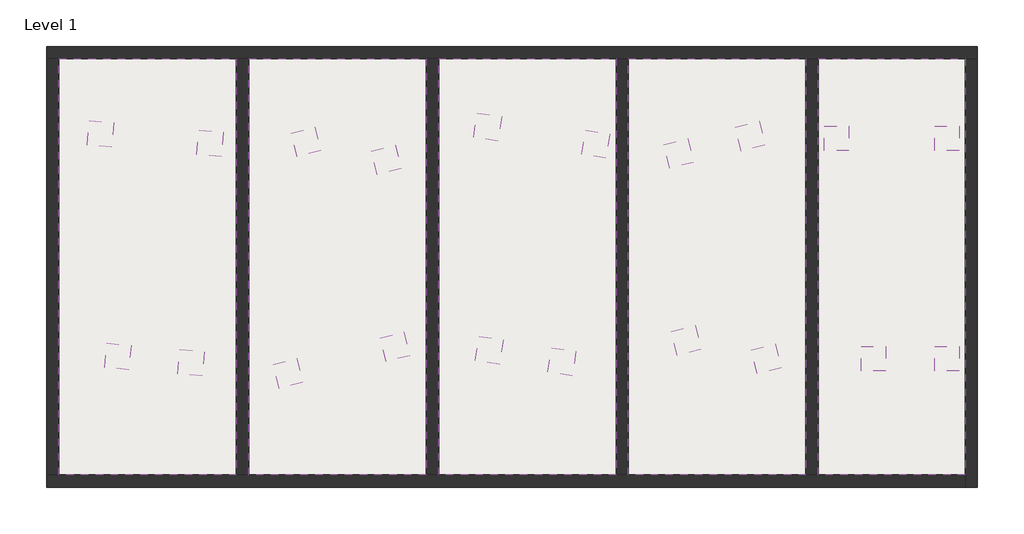
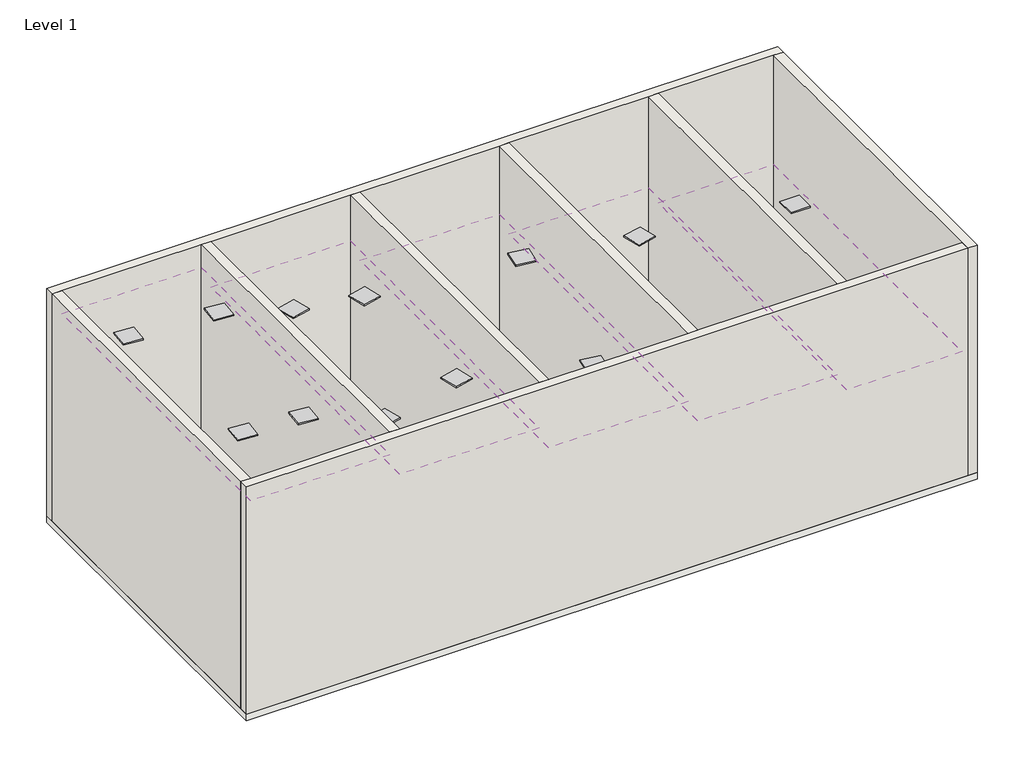
# One storey: 20 light fixtures, 8 walls, 5 coverings, 1 slab.
"""IFC4 building model written with IfcOpenShell, lengths in millimetres."""

import ifcopenshell
import ifcopenshell.guid

model = None  # the IFC model being written
_history = None  # IfcOwnerHistory: only IFC2X3 demands one
_inside = {}  # id of a spatial element -> (the spatial element, [elements in it])
_under = {}  # id of a project, library or spatial element -> (it, [spatial elements below it])
_declared = {}  # id of a project -> (the project, [libraries it declares])
_typed = {}  # id of a type object -> (the type object, [elements of that type])
_made_of = {}  # id of a material, layer set ... -> (it, [elements and type objects made of it])


def new_model(schema):
    """Start an empty IFC model of exactly this schema.

    Asked for "IFC4X3", IfcOpenShell would pick the latest addendum, in which some entities
    have other attributes; the version numbers below select the first issue.
    IFC2X3 requires an IfcOwnerHistory on every rooted entity: one is made here for all.
    """
    global model, _history
    if schema == "IFC4X3":
        model = ifcopenshell.file(schema_version=(4, 3, 0, 0))
    else:
        model = ifcopenshell.file(schema=schema)
    _inside.clear()
    _under.clear()
    _declared.clear()
    _typed.clear()
    _made_of.clear()
    _history = None
    if model.schema == "IFC2X3":
        org = make("IfcOrganization", Name="unknown")
        user = make(
            "IfcPersonAndOrganization",
            ThePerson=make("IfcPerson", FamilyName="unknown"),
            TheOrganization=org,
        )
        app = make(
            "IfcApplication",
            ApplicationDeveloper=org,
            Version="unknown",
            ApplicationFullName="unknown",
            ApplicationIdentifier="unknown",
        )
        _history = make(
            "IfcOwnerHistory",
            OwningUser=user,
            OwningApplication=app,
            ChangeAction="ADDED",
            CreationDate=0,
        )
    return model


def make(cls, **values):
    """One entity of the class cls with the attributes given. An attribute that is None is left unset."""
    return model.create_entity(
        cls, **{name: value for name, value in values.items() if value is not None}
    )


def rooted(cls, **values):
    """An entity with a GlobalId (a new one), such as an element, a storey or a relation."""
    return make(cls, GlobalId=ifcopenshell.guid.new(), OwnerHistory=_history, **values)


def si_unit(unit_type, name, prefix=None):
    """IfcSIUnit, for example si_unit("LENGTHUNIT", "METRE", prefix="MILLI")."""
    return make("IfcSIUnit", UnitType=unit_type, Prefix=prefix, Name=name)


def assignment(units):
    """IfcUnitAssignment: the units of a project."""
    return None if units is None else make("IfcUnitAssignment", Units=units)


def point(xyz):
    """IfcCartesianPoint."""
    return None if xyz is None else make("IfcCartesianPoint", Coordinates=xyz)


def direction(xyz):
    """IfcDirection."""
    return None if xyz is None else make("IfcDirection", DirectionRatios=xyz)


def frame(location, z_axis=None, x_axis=None):
    """IfcAxis2Placement3D, a coordinate frame: its origin and axes. An axis left out is left unset."""
    return make(
        "IfcAxis2Placement3D",
        Location=point(location),
        Axis=direction(z_axis),
        RefDirection=direction(x_axis),
    )


def origin():
    """The frame at (0, 0, 0) with its axes left unset."""
    return frame((0.0, 0.0, 0.0))


def origin_with_axes():
    """The frame at (0, 0, 0) with the z axis (0, 0, 1) and the x axis (1, 0, 0) written out."""
    return frame((0.0, 0.0, 0.0), z_axis=(0.0, 0.0, 1.0), x_axis=(1.0, 0.0, 0.0))


def place(relative_to, where):
    """IfcLocalPlacement: puts the frame where relative to a parent placement (None: the world)."""
    return make(
        "IfcLocalPlacement", PlacementRelTo=relative_to, RelativePlacement=where
    )


def context(
    kind, dimensions, precision=None, world=None, true_north=None, identifier=None
):
    """IfcGeometricRepresentationContext, for example the 3D "Model" context."""
    return make(
        "IfcGeometricRepresentationContext",
        ContextIdentifier=identifier,
        ContextType=kind,
        CoordinateSpaceDimension=dimensions,
        Precision=precision,
        WorldCoordinateSystem=world,
        TrueNorth=true_north,
    )


def project(units=None, contexts=None):
    """IfcProject with its units and contexts."""
    return rooted(
        "IfcProject",
        Name="project",
        RepresentationContexts=contexts,
        UnitsInContext=assignment(units),
    )


def spatial(cls, under=None, at=None, **own):
    """A site, building, storey or space (cls), placed at a placement, below another one or the project."""
    s = rooted(cls, ObjectPlacement=at, **own)
    if under is not None:
        _under.setdefault(under.id(), (under, []))[1].append(s)
    return s


def polyline(points):
    """IfcPolyline through the points."""
    return make("IfcPolyline", Points=[point(p) for p in points])


def outline(outer, holes=None, kind="AREA"):
    """IfcArbitraryClosedProfileDef: a profile drawn as a closed curve; with holes, ...WithVoids."""
    if holes is None:
        return make("IfcArbitraryClosedProfileDef", ProfileType=kind, OuterCurve=outer)
    return make(
        "IfcArbitraryProfileDefWithVoids",
        ProfileType=kind,
        OuterCurve=outer,
        InnerCurves=holes,
    )


def extrude(swept, where, along, depth):
    """IfcExtrudedAreaSolid: the profile swept, set in the frame where, extruded along a direction by depth."""
    return make(
        "IfcExtrudedAreaSolid",
        SweptArea=swept,
        Position=where,
        ExtrudedDirection=direction(along),
        Depth=depth,
    )


def faces_of(points, faces, orient=None, outer=None):
    """IfcFace entities. A face is a list of loops; a loop is a list of indices into points, from 0.

    orient and outer hold one flag for each loop. By default every Orientation is true, the
    first loop of a face is its IfcFaceOuterBound and the others are IfcFaceBound.
    """
    made = []
    for i, loops in enumerate(faces):
        bounds = []
        for j, loop in enumerate(loops):
            is_outer = j == 0 if outer is None else outer[i][j]
            bounds.append(
                make(
                    "IfcFaceOuterBound" if is_outer else "IfcFaceBound",
                    Bound=make("IfcPolyLoop", Polygon=[points[k] for k in loop]),
                    Orientation=True if orient is None else orient[i][j],
                )
            )
        made.append(make("IfcFace", Bounds=bounds))
    return made


def faceted_brep(points, faces, orient=None, outer=None, voids=None):
    """IfcFacetedBrep: a solid bounded by flat faces; with voids (closed shells), ...WithVoids."""
    shared = [point(p) for p in points]
    hull = make("IfcClosedShell", CfsFaces=faces_of(shared, faces, orient, outer))
    if voids is None:
        return make("IfcFacetedBrep", Outer=hull)
    return make(
        "IfcFacetedBrepWithVoids",
        Outer=hull,
        Voids=[
            make(cls, CfsFaces=faces_of(shared, fs, o, b)) for cls, fs, o, b in voids
        ],
    )


def shape(context_of_items, identifier, shape_type, items):
    """IfcShapeRepresentation: the items that make up one representation, for example the "Body"."""
    return make(
        "IfcShapeRepresentation",
        ContextOfItems=context_of_items,
        RepresentationIdentifier=identifier,
        RepresentationType=shape_type,
        Items=items,
    )


def source(mapping_origin, context_of_items, identifier, shape_type, items):
    """IfcRepresentationMap: a shape defined once, which mapped items show again and again."""
    return make(
        "IfcRepresentationMap",
        MappingOrigin=mapping_origin,
        MappedRepresentation=shape(context_of_items, identifier, shape_type, items),
    )


def transform(
    local_origin,
    x_axis=None,
    y_axis=None,
    z_axis=None,
    scale=None,
    scale2=None,
    scale3=None,
    uniform=True,
):
    """IfcCartesianTransformationOperator3D, or its non-uniform kind. x_axis, y_axis, z_axis: its Axis1, 2, 3."""
    if uniform:
        return make(
            "IfcCartesianTransformationOperator3D",
            Axis1=direction(x_axis),
            Axis2=direction(y_axis),
            LocalOrigin=point(local_origin),
            Scale=scale,
            Axis3=direction(z_axis),
        )
    return make(
        "IfcCartesianTransformationOperator3DnonUniform",
        Axis1=direction(x_axis),
        Axis2=direction(y_axis),
        LocalOrigin=point(local_origin),
        Scale=scale,
        Axis3=direction(z_axis),
        Scale2=scale2,
        Scale3=scale3,
    )


def mapped(mapping_source, mapping_target):
    """IfcMappedItem: shows the shape of a source again, moved by a transform."""
    return make(
        "IfcMappedItem", MappingSource=mapping_source, MappingTarget=mapping_target
    )


def made_of(thing, what):
    """Note that an element or type object is made of a material, layer set ...; save() writes the relation."""
    if what is not None:
        _made_of.setdefault(what.id(), (what, []))[1].append(thing)
    return thing


def element(
    cls,
    number,
    at=None,
    inside=None,
    cuts=None,
    type_object=None,
    material=None,
    context=None,
    identifier="Body",
    shape_type=None,
    held_by="IfcProductDefinitionShape",
    body=None,
    shapes=None,
    **own,
):
    """One element of the class cls, such as IfcWall. Its Tag is "e" and its number.

    at: its placement. inside: the storey or other place that contains it. cuts: it is an
    opening in that element (IfcRelVoidsElement). A single representation is given by context,
    identifier, shape_type and body (its items); several are given by shapes. held_by: the class
    of the entity that holds the representations. save() writes the other relations.
    """
    e = rooted(cls, Tag="e%d" % number, ObjectPlacement=at, **own)
    if body is not None:
        shapes = [shape(context, identifier, shape_type, body)]
    if shapes is not None:
        e.Representation = make(held_by, Representations=shapes)
    if inside is not None:
        _inside.setdefault(inside.id(), (inside, []))[1].append(e)
    if cuts is not None:
        rooted(
            "IfcRelVoidsElement", RelatingBuildingElement=cuts, RelatedOpeningElement=e
        )
    if type_object is not None:
        _typed.setdefault(type_object.id(), (type_object, []))[1].append(e)
    return made_of(e, material)


def aggregate(whole, parts):
    """IfcRelAggregates: a whole, such as a stair, and the parts it consists of."""
    return rooted("IfcRelAggregates", RelatingObject=whole, RelatedObjects=parts)


def save(model, path):
    """Write the relations noted so far, then the file.

    IfcRelAggregates (storeys below a building ...), IfcRelContainedInSpatialStructure (elements
    in a storey), IfcRelDefinesByType, IfcRelAssociatesMaterial and IfcRelDeclares: one each for
    every whole, place, type object, material and project.
    """
    for whole, parts in _under.values():
        aggregate(whole, parts)
    for where, things in _inside.values():
        rooted(
            "IfcRelContainedInSpatialStructure",
            RelatedElements=things,
            RelatingStructure=where,
        )
    for kind, things in _typed.values():
        rooted("IfcRelDefinesByType", RelatedObjects=things, RelatingType=kind)
    for what, things in _made_of.values():
        rooted("IfcRelAssociatesMaterial", RelatedObjects=things, RelatingMaterial=what)
    for by, libraries in _declared.values():
        rooted("IfcRelDeclares", RelatingContext=by, RelatedDefinitions=libraries)
    model.write(path)


def downlight_downlight_20077eaa(model_context):
    return source(origin(), model_context, "Body", "SweptSolid", [
        extrude(outline(polyline([(200.0, -200.0), (-200.0, -200.0), (-200.0, 200.0), (200.0, 200.0), (200.0, -200.0)])), frame((0.0, 0.0, -4.6872227), z_axis=(0.0, 0.0, 1.0), x_axis=(1.0, 0.0, 0.0)), (0.0, 0.0, 1.0), 24.9370919),
    ])


model = new_model("IFC4")

# Units and contexts
model_context = context("Model", 3, world=origin())
ifc_project = project(units=[si_unit("LENGTHUNIT", "METRE", prefix="MILLI")], contexts=[model_context])

# Site, building, storey
site = spatial("IfcSite", under=ifc_project)
building = spatial("IfcBuilding", under=site)
storey = spatial("IfcBuildingStorey", under=building, Name="Level 1", Elevation=0.0)

# Coverings
placement = place(None, origin())
element("IfcCovering", 1, ObjectType="600 x 600mm Grid", at=placement, inside=storey, context=model_context, shape_type="SweptSolid", body=[
    extrude(outline(polyline([(4711.6370984, -2494.7382368), (4711.6370984, 4305.2617632), (7111.6370984, 4305.2617632), (7111.6370984, -2494.7382368), (4711.6370984, -2494.7382368)])), frame((0.0, 0.0, 2600.0), z_axis=(0.0, 0.0, 1.0), x_axis=(1.0, 0.0, 0.0)), (0.0, 0.0, 1.0), 52.0),
])
element("IfcCovering", 2, ObjectType="600 x 600mm Grid", at=placement, inside=storey, context=model_context, shape_type="SweptSolid", body=[
    extrude(outline(polyline([(1611.6370984, -2494.7382368), (1611.6370984, 4305.2617632), (4511.6370984, 4305.2617632), (4511.6370984, -2494.7382368), (1611.6370984, -2494.7382368)])), frame((0.0, 0.0, 3000.0), z_axis=(0.0, 0.0, 1.0), x_axis=(1.0, 0.0, 0.0)), (0.0, 0.0, 1.0), 52.0),
])
element("IfcCovering", 3, ObjectType="600 x 600mm Grid", at=placement, inside=storey, context=model_context, shape_type="SweptSolid", body=[
    extrude(outline(polyline([(-1488.3629016, -2494.7382368), (-1488.3629016, 4305.2617632), (1411.6370984, 4305.2617632), (1411.6370984, -2494.7382368), (-1488.3629016, -2494.7382368)])), frame((0.0, 0.0, 3500.0), z_axis=(0.0, 0.0, 1.0), x_axis=(1.0, 0.0, 0.0)), (0.0, 0.0, 1.0), 52.0),
])
element("IfcCovering", 4, ObjectType="600 x 600mm Grid", at=placement, inside=storey, context=model_context, shape_type="SweptSolid", body=[
    extrude(outline(polyline([(-4588.3629016, -2494.7382368), (-4588.3629016, 4305.2617632), (-1688.3629016, 4305.2617632), (-1688.3629016, -2494.7382368), (-4588.3629016, -2494.7382368)])), frame((0.0, 0.0, 4000.0), z_axis=(0.0, 0.0, 1.0), x_axis=(1.0, 0.0, 0.0)), (0.0, 0.0, 1.0), 52.0),
])
element("IfcCovering", 5, ObjectType="600 x 600mm Grid", at=placement, inside=storey, context=model_context, shape_type="SweptSolid", body=[
    extrude(outline(polyline([(-7688.3629016, 4305.2617632), (-4788.3629016, 4305.2617632), (-4788.3629016, -2494.7382368), (-7688.3629016, -2494.7382368), (-7688.3629016, 4305.2617632)])), frame((0.0, 0.0, 4500.0), z_axis=(0.0, 0.0, 1.0), x_axis=(1.0, 0.0, 0.0)), (0.0, 0.0, 1.0), 52.0),
])

# Light fixtures
downlight_downlight_shape = downlight_downlight_20077eaa(model_context)
element("IfcLightFixture", 6, ObjectType="Downlight : Downlight", at=placement, inside=storey, context=model_context, shape_type="MappedRepresentation", body=[
    mapped(downlight_downlight_shape, transform((-7009.3072235, 3078.2167678, 4500.0), x_axis=(0.9961946980917439, -0.08715574274767758, 0.0), y_axis=(0.08715574274767758, 0.9961946980917439, 0.0), z_axis=(0.0, 0.0, 1.0))),
])
element("IfcLightFixture", 7, ObjectType="Downlight : Downlight", at=placement, inside=storey, context=model_context, shape_type="MappedRepresentation", body=[
    mapped(downlight_downlight_shape, transform((-5216.1567669, 2921.3364309, 4500.0), x_axis=(0.9961946980917439, -0.08715574274767879, 0.0), y_axis=(0.08715574274767879, 0.9961946980917439, 0.0), z_axis=(0.0, 0.0, 1.0))),
])
element("IfcLightFixture", 8, ObjectType="Downlight : Downlight", at=placement, inside=storey, context=model_context, shape_type="MappedRepresentation", body=[
    mapped(downlight_downlight_shape, transform((-5529.9174408, -664.9644822, 4500.0), x_axis=(0.9961946980917413, -0.08715574274770704, 0.0), y_axis=(0.08715574274770704, 0.9961946980917413, 0.0), z_axis=(0.0, 0.0, 1.0))),
])
element("IfcLightFixture", 9, ObjectType="Downlight : Downlight", at=placement, inside=storey, context=model_context, shape_type="MappedRepresentation", body=[
    mapped(downlight_downlight_shape, transform((-6725.3510785, -560.3775909, 4500.0), x_axis=(0.9961946980917413, -0.08715574274770621, 0.0), y_axis=(0.08715574274770621, 0.9961946980917413, 0.0), z_axis=(0.0, 0.0, 1.0))),
])
element("IfcLightFixture", 10, ObjectType="Downlight : Downlight", at=placement, inside=storey, context=model_context, shape_type="MappedRepresentation", body=[
    mapped(downlight_downlight_shape, transform((-3651.9813594, 2945.0444871, 4000.0), x_axis=(0.24192189559968028, -0.9702957262759934, 0.0), y_axis=(0.9702957262759934, 0.24192189559968028, 0.0), z_axis=(0.0, 0.0, 1.0))),
])
element("IfcLightFixture", 11, ObjectType="Downlight : Downlight", at=placement, inside=storey, context=model_context, shape_type="MappedRepresentation", body=[
    mapped(downlight_downlight_shape, transform((-2342.4733505, 2653.173326, 4000.0), x_axis=(0.24192189559967206, -0.9702957262759955, 0.0), y_axis=(0.9702957262759955, 0.24192189559967206, 0.0), z_axis=(0.0, 0.0, 1.0))),
])
element("IfcLightFixture", 12, ObjectType="Downlight : Downlight", at=placement, inside=storey, context=model_context, shape_type="MappedRepresentation", body=[
    mapped(downlight_downlight_shape, transform((-2198.8850995, -402.8669901, 4000.0), x_axis=(0.24192189559958152, -0.970295726276018, 0.0), y_axis=(0.970295726276018, 0.24192189559958152, 0.0), z_axis=(0.0, 0.0, 1.0))),
])
element("IfcLightFixture", 13, ObjectType="Downlight : Downlight", at=placement, inside=storey, context=model_context, shape_type="MappedRepresentation", body=[
    mapped(downlight_downlight_shape, transform((-3945.4174068, -838.3264022, 4000.0), x_axis=(0.241921895599675, -0.9702957262759947, 0.0), y_axis=(0.9702957262759947, 0.241921895599675, 0.0), z_axis=(0.0, 0.0, 1.0))),
])
element("IfcLightFixture", 14, ObjectType="Downlight : Downlight", at=placement, inside=storey, context=model_context, shape_type="MappedRepresentation", body=[
    mapped(downlight_downlight_shape, transform((-687.666432, 3190.6624322, 3500.0), x_axis=(0.9876883405951378, -0.15643446504023112, 0.0), y_axis=(0.15643446504023112, 0.9876883405951378, 0.0), z_axis=(0.0, 0.0, 1.0))),
])
element("IfcLightFixture", 15, ObjectType="Downlight : Downlight", at=placement, inside=storey, context=model_context, shape_type="MappedRepresentation", body=[
    mapped(downlight_downlight_shape, transform((1079.2864189, 2909.0803951, 3500.0), x_axis=(0.9876883405951377, -0.15643446504023206, 0.0), y_axis=(0.15643446504023206, 0.9876883405951377, 0.0), z_axis=(0.0, 0.0, 1.0))),
])
element("IfcLightFixture", 16, ObjectType="Downlight : Downlight", at=placement, inside=storey, context=model_context, shape_type="MappedRepresentation", body=[
    mapped(downlight_downlight_shape, transform((527.0085069, -646.597631, 3500.0), x_axis=(0.9876883405951323, -0.15643446504026584, 0.0), y_axis=(0.15643446504026584, 0.9876883405951323, 0.0), z_axis=(0.0, 0.0, 1.0))),
])
element("IfcLightFixture", 17, ObjectType="Downlight : Downlight", at=placement, inside=storey, context=model_context, shape_type="MappedRepresentation", body=[
    mapped(downlight_downlight_shape, transform((-658.2175018, -458.876273, 3500.0), x_axis=(0.9876883405951323, -0.15643446504026556, 0.0), y_axis=(0.15643446504026556, 0.9876883405951323, 0.0), z_axis=(0.0, 0.0, 1.0))),
])
element("IfcLightFixture", 18, ObjectType="Downlight : Downlight", at=placement, inside=storey, context=model_context, shape_type="MappedRepresentation", body=[
    mapped(downlight_downlight_shape, transform((2433.0525413, 2757.895041, 3000.0), x_axis=(0.2353878351035713, -0.9719015212897107, 0.0), y_axis=(0.9719015212897107, 0.2353878351035713, 0.0), z_axis=(0.0, 0.0, 1.0))),
])
element("IfcLightFixture", 19, ObjectType="Downlight : Downlight", at=placement, inside=storey, context=model_context, shape_type="MappedRepresentation", body=[
    mapped(downlight_downlight_shape, transform((3599.3343668, 3040.3604431, 3000.0), x_axis=(0.235387835103798, -0.9719015212896558, 0.0), y_axis=(0.9719015212896558, 0.235387835103798, 0.0), z_axis=(0.0, 0.0, 1.0))),
])
element("IfcLightFixture", 20, ObjectType="Downlight : Downlight", at=placement, inside=storey, context=model_context, shape_type="MappedRepresentation", body=[
    mapped(downlight_downlight_shape, transform((3863.5896604, -599.7177346, 3000.0), x_axis=(0.23538783510367559, -0.9719015212896854, 0.0), y_axis=(0.9719015212896854, 0.23538783510367559, 0.0), z_axis=(0.0, 0.0, 1.0))),
])
element("IfcLightFixture", 21, ObjectType="Downlight : Downlight", at=placement, inside=storey, context=model_context, shape_type="MappedRepresentation", body=[
    mapped(downlight_downlight_shape, transform((2556.0751338, -299.042224, 3000.0), x_axis=(0.23538783510357353, -0.9719015212897102, 0.0), y_axis=(0.9719015212897102, 0.23538783510357353, 0.0), z_axis=(0.0, 0.0, 1.0))),
])
element("IfcLightFixture", 22, ObjectType="Downlight : Downlight", at=placement, inside=storey, context=model_context, shape_type="MappedRepresentation", body=[
    mapped(downlight_downlight_shape, transform((5011.6370984, 3005.2617632, 2600.0), x_axis=(1.0, 0.0, 0.0), y_axis=(0.0, 1.0, 0.0), z_axis=(0.0, 0.0, 1.0))),
])
element("IfcLightFixture", 23, ObjectType="Downlight : Downlight", at=placement, inside=storey, context=model_context, shape_type="MappedRepresentation", body=[
    mapped(downlight_downlight_shape, transform((6811.6370984, 3005.2617632, 2600.0), x_axis=(1.0, 0.0, 0.0), y_axis=(0.0, 1.0, 0.0), z_axis=(0.0, 0.0, 1.0))),
])
element("IfcLightFixture", 24, ObjectType="Downlight : Downlight", at=placement, inside=storey, context=model_context, shape_type="MappedRepresentation", body=[
    mapped(downlight_downlight_shape, transform((6811.6370984, -594.7382368, 2600.0), x_axis=(1.0, 0.0, 0.0), y_axis=(0.0, 1.0, 0.0), z_axis=(0.0, 0.0, 1.0))),
])
element("IfcLightFixture", 25, ObjectType="Downlight : Downlight", at=placement, inside=storey, context=model_context, shape_type="MappedRepresentation", body=[
    mapped(downlight_downlight_shape, transform((5611.6370984, -594.7382368, 2600.0), x_axis=(1.0, 0.0, 0.0), y_axis=(0.0, 1.0, 0.0), z_axis=(0.0, 0.0, 1.0))),
])

# Slab
element("IfcSlab", 26, ObjectType="Generic 150mm", at=placement, inside=storey, context=model_context, shape_type="SweptSolid", body=[
    extrude(outline(polyline([(7311.6370984, 4505.2617632), (7311.6370984, -2694.7382368), (-7888.3629016, -2694.7382368), (-7888.3629016, 4505.2617632), (7311.6370984, 4505.2617632)])), frame((0.0, 0.0, -150.0), z_axis=(0.0, 0.0, 1.0), x_axis=(1.0, 0.0, 0.0)), (0.0, 0.0, 1.0), 150.0),
])

# Walls
element("IfcWall", 27, ObjectType="Generic - 200mm", at=placement, inside=storey, context=model_context, shape_type="Brep", body=[
    faceted_brep([(-7888.3629016, 4305.2617632, 0.0), (-7688.3629016, 4305.2617632, 0.0), (-4788.3629016, 4305.2617632, 0.0), (-4588.3629016, 4305.2617632, 0.0), (-1688.3629016, 4305.2617632, 0.0), (-1488.3629016, 4305.2617632, 0.0), (1411.6370984, 4305.2617632, 0.0), (1611.6370984, 4305.2617632, 0.0), (4511.6370984, 4305.2617632, 0.0), (4711.6370984, 4305.2617632, 0.0), (7111.6370984, 4305.2617632, 0.0), (7311.6370984, 4305.2617632, 0.0), (7311.6370984, 4305.2617632, 5000.0), (7111.6370984, 4305.2617632, 5000.0), (4711.6370984, 4305.2617632, 5000.0), (4511.6370984, 4305.2617632, 5000.0), (1611.6370984, 4305.2617632, 5000.0), (1411.6370984, 4305.2617632, 5000.0), (-1488.3629016, 4305.2617632, 5000.0), (-1688.3629016, 4305.2617632, 5000.0), (-4588.3629016, 4305.2617632, 5000.0), (-4788.3629016, 4305.2617632, 5000.0), (-7688.3629016, 4305.2617632, 5000.0), (-7888.3629016, 4305.2617632, 5000.0), (-7888.3629016, 4505.2617632, 0.0), (-7888.3629016, 4505.2617632, 5000.0), (7311.6370984, 4505.2617632, 5000.0), (7311.6370984, 4505.2617632, 0.0)], [[[0, 1, 2, 3, 4, 5, 6, 7, 8, 9, 10, 11, 12, 13, 14, 15, 16, 17, 18, 19, 20, 21, 22, 23]], [[24, 25, 26, 27]], [[11, 10, 9, 8, 7, 6, 5, 4, 3, 2, 1, 0, 24, 27]], [[23, 22, 21, 20, 19, 18, 17, 16, 15, 14, 13, 12, 26, 25]], [[12, 11, 27, 26]], [[0, 23, 25, 24]]]),
])
element("IfcWall", 28, ObjectType="Generic - 200mm", at=placement, inside=storey, context=model_context, shape_type="Brep", body=[
    faceted_brep([(7111.6370984, 4305.2617632, 0.0), (7111.6370984, -2494.7382368, 0.0), (7111.6370984, -2694.7382368, 0.0), (7111.6370984, -2694.7382368, 5000.0), (7111.6370984, -2494.7382368, 5000.0), (7111.6370984, 4305.2617632, 5000.0), (7311.6370984, 4305.2617632, 0.0), (7311.6370984, 4305.2617632, 5000.0), (7311.6370984, -2694.7382368, 5000.0), (7311.6370984, -2694.7382368, 0.0)], [[[0, 1, 2, 3, 4, 5]], [[6, 7, 8, 9]], [[2, 1, 0, 6, 9]], [[5, 4, 3, 8, 7]], [[0, 5, 7, 6]], [[3, 2, 9, 8]]]),
])
element("IfcWall", 29, ObjectType="Generic - 200mm", at=placement, inside=storey, context=model_context, shape_type="Brep", body=[
    faceted_brep([(7111.6370984, -2494.7382368, 0.0), (4711.6370984, -2494.7382368, 0.0), (4511.6370984, -2494.7382368, 0.0), (1611.6370984, -2494.7382368, 0.0), (1411.6370984, -2494.7382368, 0.0), (-1488.3629016, -2494.7382368, 0.0), (-1688.3629016, -2494.7382368, 0.0), (-4588.3629016, -2494.7382368, 0.0), (-4788.3629016, -2494.7382368, 0.0), (-7688.3629016, -2494.7382368, 0.0), (-7888.3629016, -2494.7382368, 0.0), (-7888.3629016, -2494.7382368, 5000.0), (-7688.3629016, -2494.7382368, 5000.0), (-4788.3629016, -2494.7382368, 5000.0), (-4588.3629016, -2494.7382368, 5000.0), (-1688.3629016, -2494.7382368, 5000.0), (-1488.3629016, -2494.7382368, 5000.0), (1411.6370984, -2494.7382368, 5000.0), (1611.6370984, -2494.7382368, 5000.0), (4511.6370984, -2494.7382368, 5000.0), (4711.6370984, -2494.7382368, 5000.0), (7111.6370984, -2494.7382368, 5000.0), (7111.6370984, -2694.7382368, 0.0), (7111.6370984, -2694.7382368, 5000.0), (-7888.3629016, -2694.7382368, 5000.0), (-7888.3629016, -2694.7382368, 0.0)], [[[0, 1, 2, 3, 4, 5, 6, 7, 8, 9, 10, 11, 12, 13, 14, 15, 16, 17, 18, 19, 20, 21]], [[22, 23, 24, 25]], [[10, 9, 8, 7, 6, 5, 4, 3, 2, 1, 0, 22, 25]], [[21, 20, 19, 18, 17, 16, 15, 14, 13, 12, 11, 24, 23]], [[0, 21, 23, 22]], [[11, 10, 25, 24]]]),
])
element("IfcWall", 30, ObjectType="Generic - 200mm", at=placement, inside=storey, context=model_context, shape_type="SweptSolid", body=[
    extrude(outline(polyline([(-7688.3629016, 4305.2617632), (-7688.3629016, -2494.7382368), (-7888.3629016, -2494.7382368), (-7888.3629016, 4305.2617632), (-7688.3629016, 4305.2617632)])), origin_with_axes(), (0.0, 0.0, 1.0), 5000.0),
])
element("IfcWall", 31, ObjectType="Generic - 200mm", at=placement, inside=storey, context=model_context, shape_type="SweptSolid", body=[
    extrude(outline(polyline([(-4788.3629016, -2494.7382368), (-4788.3629016, 4305.2617632), (-4588.3629016, 4305.2617632), (-4588.3629016, -2494.7382368), (-4788.3629016, -2494.7382368)])), origin_with_axes(), (0.0, 0.0, 1.0), 5000.0),
])
element("IfcWall", 32, ObjectType="Generic - 200mm", at=placement, inside=storey, context=model_context, shape_type="SweptSolid", body=[
    extrude(outline(polyline([(-1688.3629016, -2494.7382368), (-1688.3629016, 4305.2617632), (-1488.3629016, 4305.2617632), (-1488.3629016, -2494.7382368), (-1688.3629016, -2494.7382368)])), origin_with_axes(), (0.0, 0.0, 1.0), 5000.0),
])
element("IfcWall", 33, ObjectType="Generic - 200mm", at=placement, inside=storey, context=model_context, shape_type="SweptSolid", body=[
    extrude(outline(polyline([(1411.6370984, -2494.7382368), (1411.6370984, 4305.2617632), (1611.6370984, 4305.2617632), (1611.6370984, -2494.7382368), (1411.6370984, -2494.7382368)])), origin_with_axes(), (0.0, 0.0, 1.0), 5000.0),
])
element("IfcWall", 34, ObjectType="Generic - 200mm", at=placement, inside=storey, context=model_context, shape_type="SweptSolid", body=[
    extrude(outline(polyline([(4511.6370984, -2494.7382368), (4511.6370984, 4305.2617632), (4711.6370984, 4305.2617632), (4711.6370984, -2494.7382368), (4511.6370984, -2494.7382368)])), origin_with_axes(), (0.0, 0.0, 1.0), 5000.0),
])

save(model, "model.ifc")

# Revit data of these elements
# Project information
#   Project Issue Date = "Issue Date"
#   Project Status = "Project Status"
#   Client Name = "Owner"
#   Project Address = "Enter address here"
#   Project Name = "Project Name"
#   Project Number = "0001"
# Type "600 x 600mm Grid"
#   built-in parameter 1002203 = 1 (stored number, unit not read)
#   built-in parameter 1002202 = 1 (stored number, unit not read)
#   Layers, outside or top first: 0.036 m "Default" (function 1); 0.016 m "Ceiling Tile 600 x 600" (function 5)
# Type "Downlight : Downlight"
#   Default Elevation = 0
# Type "Generic 150mm"
#   Function = 0
#   Layers, outside or top first: 0.15 m no material (function 1)
# Type "Generic - 200mm"
#   Layers, outside or top first: 0.2 m no material (function 1)
# Element 1 (IfcCovering, "600 x 600mm Grid")
#   Height Offset From Level = 2.6 m
#   Phase Created = New Construction
#   Materials on its faces: "Ceiling Tile 600 x 600", "Default"
# Element 2 (IfcCovering, "600 x 600mm Grid")
#   Height Offset From Level = 3 m
#   Phase Created = New Construction
#   Materials on its faces: "Ceiling Tile 600 x 600", "Default"
# Element 3 (IfcCovering, "600 x 600mm Grid")
#   Height Offset From Level = 3.5 m
#   Phase Created = New Construction
#   Materials on its faces: "Ceiling Tile 600 x 600", "Default"
# Element 4 (IfcCovering, "600 x 600mm Grid")
#   Height Offset From Level = 4 m
#   Phase Created = New Construction
#   Materials on its faces: "Ceiling Tile 600 x 600", "Default"
# Element 5 (IfcCovering, "600 x 600mm Grid")
#   Height Offset From Level = 4.5 m
#   Phase Created = New Construction
#   Materials on its faces: "Ceiling Tile 600 x 600", "Default"
# Element 6 (IfcLightFixture, "Downlight : Downlight")
#   Mark = "24"
#   Phase Created = New Construction
# Element 7 (IfcLightFixture, "Downlight : Downlight")
#   Mark = "55"
#   Phase Created = New Construction
# Element 8 (IfcLightFixture, "Downlight : Downlight")
#   Mark = "56"
#   Phase Created = New Construction
# Element 9 (IfcLightFixture, "Downlight : Downlight")
#   Mark = "57"
#   Phase Created = New Construction
# Element 10 (IfcLightFixture, "Downlight : Downlight")
#   Mark = "58"
#   Phase Created = New Construction
# Element 11 (IfcLightFixture, "Downlight : Downlight")
#   Mark = "59"
#   Phase Created = New Construction
# Element 12 (IfcLightFixture, "Downlight : Downlight")
#   Mark = "60"
#   Phase Created = New Construction
# Element 13 (IfcLightFixture, "Downlight : Downlight")
#   Mark = "61"
#   Phase Created = New Construction
# Element 14 (IfcLightFixture, "Downlight : Downlight")
#   Mark = "62"
#   Phase Created = New Construction
# Element 15 (IfcLightFixture, "Downlight : Downlight")
#   Mark = "63"
#   Phase Created = New Construction
# Element 16 (IfcLightFixture, "Downlight : Downlight")
#   Mark = "64"
#   Phase Created = New Construction
# Element 17 (IfcLightFixture, "Downlight : Downlight")
#   Mark = "65"
#   Phase Created = New Construction
# Element 18 (IfcLightFixture, "Downlight : Downlight")
#   Mark = "66"
#   Phase Created = New Construction
# Element 19 (IfcLightFixture, "Downlight : Downlight")
#   Mark = "67"
#   Phase Created = New Construction
# Element 20 (IfcLightFixture, "Downlight : Downlight")
#   Mark = "68"
#   Phase Created = New Construction
# Element 21 (IfcLightFixture, "Downlight : Downlight")
#   Mark = "69"
#   Phase Created = New Construction
# Element 22 (IfcLightFixture, "Downlight : Downlight")
#   Mark = "70"
#   Phase Created = New Construction
# Element 23 (IfcLightFixture, "Downlight : Downlight")
#   Mark = "71"
#   Phase Created = New Construction
# Element 24 (IfcLightFixture, "Downlight : Downlight")
#   Mark = "72"
#   Phase Created = New Construction
# Element 25 (IfcLightFixture, "Downlight : Downlight")
#   Mark = "73"
#   Phase Created = New Construction
# Element 26 (IfcSlab, "Generic 150mm")
#   Height Offset From Level = 0 m
#   Phase Created = New Construction
#   Materials on its faces: "Default Floor"
# Elements 27, 28, 29, 30, 31, 32, 33, 34 (IfcWall, "Generic - 200mm")
#   Top Offset = 0 m
#   Base Offset = 0 m
#   wall height = 5 m
#   Phase Created = New Construction
#   Base Constraint = Level 1
#   Top Constraint = Level 2
#   Materials on its faces: "Default Wall"
# Materials
#   "Default": class "Generic", colour RGB 127 127 127, transparency 0, Cost = 0
#   "Ceiling Tile 600 x 600": class "Generic", colour RGB 235 235 235, transparency 0, Description = "Acoustic ceiling tile", Cost = 0
#   "Default Floor": class "Miscellaneous", colour RGB 127 127 127, transparency 0, Cost = 0
#   "Default Wall": class "Miscellaneous", colour RGB 128 128 128, transparency 0, Cost = 0
